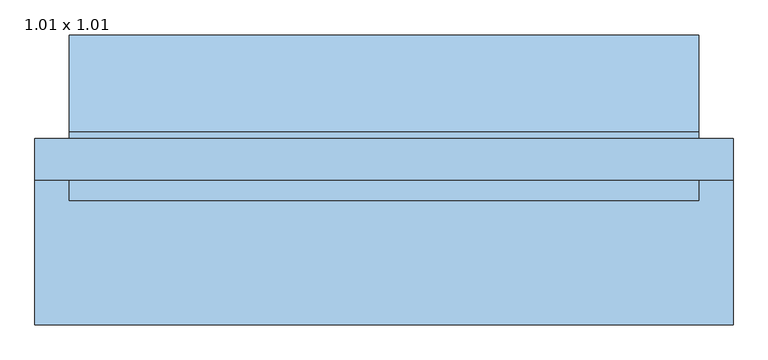
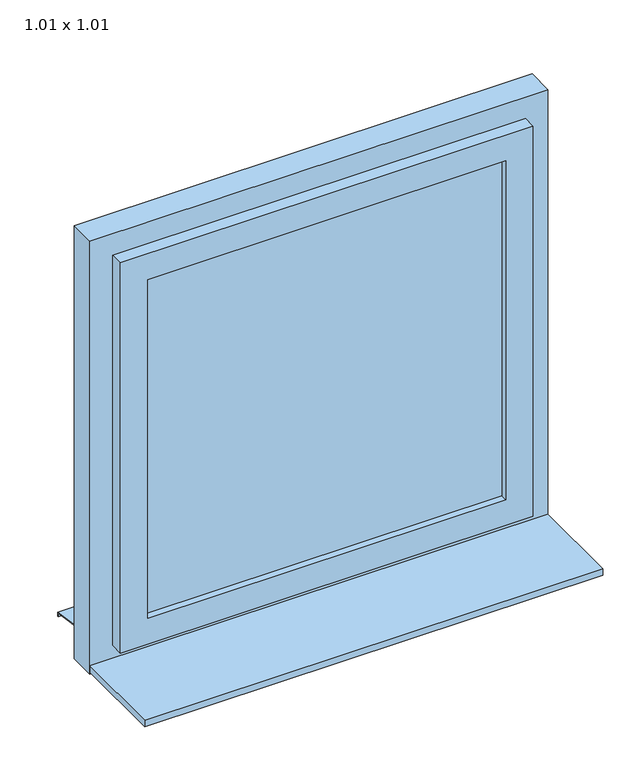
"""IFC4 building model written with IfcOpenShell, lengths in millimetres: window geometry, Fenster 1-flg - Anschlag : 1.01 x 1.01."""

from ifc_helpers import new_model, si_unit, frame, origin, place, context, project, spatial, polyline, outline, extrude, faceted_brep, source, transform, mapped, element, save


def window_1_01_x_1_01_b7243dc8(model_context):
    return source(origin(), model_context, "Body", "SolidModel", [
        extrude(outline(polyline([(-525.0, -210.0), (-525.0, 0.0), (485.0, 0.0), (485.0, -210.0), (-525.0, -210.0)])), frame((0.0, 0.0, 1005.0), z_axis=(0.0, 0.0, 1.0), x_axis=(1.0, 0.0, 0.0)), (0.0, 0.0, 1.0), 15.0),
        extrude(outline(polyline([(375.0, -15.0), (-415.0, -15.0), (-415.0, 15.0), (375.0, 15.0), (375.0, -15.0)])), frame((0.0, 0.0, 1110.0), z_axis=(0.0, 0.0, 1.0), x_axis=(1.0, 0.0, 0.0)), (0.0, 0.0, 1.0), 790.0),
        extrude(outline(polyline([(70.0221543, 1020.0), (210.0, 1000.0), (210.0, 990.0), (208.0, 990.0), (208.0, 998.3604634), (69.8240723, 1018.0), (60.0, 1018.0), (60.0, 1020.0), (70.0221543, 1020.0)])), frame((-475.0, 0.0, 0.0), z_axis=(1.0, 0.0, 0.0), x_axis=(0.0, 1.0, 0.0)), (0.0, 0.0, 1.0), 910.0),
        extrude(outline(polyline([(2010.0, 485.0), (2010.0, -525.0), (1000.0, -525.0), (1000.0, 485.0), (2010.0, 485.0)]), holes=[polyline([(1930.0, 405.0), (1080.0, 405.0), (1080.0, -445.0), (1930.0, -445.0), (1930.0, 405.0)])]), frame((0.0, 0.0, 0.0), z_axis=(0.0, 1.0, 0.0), x_axis=(0.0, 0.0, 1.0)), (0.0, 0.0, 1.0), 60.0),
        faceted_brep([(435.0, 0.0, 1960.0), (435.0, -30.0, 1960.0), (435.0, -30.0, 1050.0), (435.0, 0.0, 1050.0), (-475.0, -30.0, 1960.0), (-475.0, -30.0, 1050.0), (375.0, -30.0, 1110.0), (-415.0, -30.0, 1110.0), (-415.0, -30.0, 1900.0), (375.0, -30.0, 1900.0), (-475.0, 0.0, 1050.0), (-475.0, 0.0, 1960.0), (405.0, 0.0, 1930.0), (-445.0, 0.0, 1930.0), (-445.0, 0.0, 1080.0), (405.0, 0.0, 1080.0), (405.0, 30.0, 1930.0), (405.0, 30.0, 1080.0), (-445.0, 30.0, 1080.0), (-445.0, 30.0, 1930.0), (375.0, 30.0, 1900.0), (-415.0, 30.0, 1900.0), (-415.0, 30.0, 1110.0), (375.0, 30.0, 1110.0)], [[[0, 1, 2, 3]], [[1, 4, 5, 2], [6, 7, 8, 9]], [[3, 2, 5, 10]], [[3, 10, 11, 0], [12, 13, 14, 15]], [[16, 12, 15, 17]], [[17, 15, 14, 18]], [[17, 18, 19, 16], [20, 21, 22, 23]], [[9, 20, 23, 6]], [[6, 23, 22, 7]], [[10, 5, 4, 11]], [[18, 14, 13, 19]], [[7, 22, 21, 8]], [[11, 4, 1, 0]], [[19, 13, 12, 16]], [[8, 21, 20, 9]]]),
    ])


if __name__ == "__main__":
    model = new_model("IFC4")
    model_context = context("Model", 3, world=origin())
    ifc_project = project(units=[si_unit("LENGTHUNIT", "METRE", prefix="MILLI")], contexts=[model_context])
    site = spatial("IfcSite", under=ifc_project)
    building = spatial("IfcBuilding", under=site)
    placement = place(None, origin())
    window_1_01_x_1_01_shape = window_1_01_x_1_01_b7243dc8(model_context)
    element("IfcWindow", 1, ObjectType="Fenster 1-flg - Anschlag : 1.01 x 1.01", at=placement, inside=building, context=model_context, shape_type="MappedRepresentation", body=[
        mapped(window_1_01_x_1_01_shape, transform((0.0, 0.0, 0.0), x_axis=(1.0, 0.0, 0.0), y_axis=(0.0, 1.0, 0.0), z_axis=(0.0, 0.0, 1.0))),
    ])
    save(model, "model.ifc")

# Revit data of these elements
# Type "Fenster 1-flg - Anschlag : 1.01 x 1.01"
#   Type Mark = "47"
#   Operation = "SinglePanel"
#   Keynote = "16.05.01"
#   Construction Type Id = "GSP4R"
#   Analytic Construction = "1/8 Zoll Pilkington-Verglasung einfach"
#   Visual Light Transmittance = 0.9
#   Thermal Resistance (R) = 0.1491 (m²·K)/W
#   Solar Heat Gain Coefficient = 0.86
#   Anschlagsbreite seitlich = 0.050 m
#   Rough Width = 1.010 m
#   Rough Height = 1.010 m
#   Heat Transfer Coefficient (U) = 6.7069 W/(m²·K)
#   Rahmentiefe = 0.060 m
#   Rahmenhöhe unten = 0.080 m
#   Rahmenhöhe oben = 0.080 m
#   Rahmenbreite = 0.080 m
#   Height = 1.010 m
#   Flügeltiefe = 0.060 m
#   Flügelbreite = 0.060 m
#   Einbautiefe (von außen) [instance default] = 0.120 m
#   Width = 1.010 m
#   Anschlagsbreite oben = 0.050 m
#   Klappflügel [instance default] = no
#   Öffnungsrichtung oben [instance default] = yes
#   Öffnungsrichtung in Draufsicht anzeigen [instance default] = no
#   Drehflügel [instance default] = yes
#   Rahmen [instance default] = none
#   Glas [instance default] = none
#   Flügel [instance default] = none
#   Fensterbank innen [instance default] = none
#   Fensterbank außen [instance default] = none
#   Wall Closure = (empty or 0)
# Element 1 (IfcWindow, "Fenster 1-flg - Anschlag : 1.01 x 1.01")
#   Materials on its faces: "Kunststoff - Weiß", "Holz - Birke", "Glas"
# Materials
#   "Kunststoff - Weiß": class "Kunststoff", colour RGB 249 249 249, transparency 0
#   "Holz - Birke": class "Holz", colour RGB 213 164 103, transparency 0
#   "Glas": class "Glas", colour RGB 0 0 255, transparency 0.75, Comments = "Renderdarstellung nicht aktualisiert ", Cost = 0
